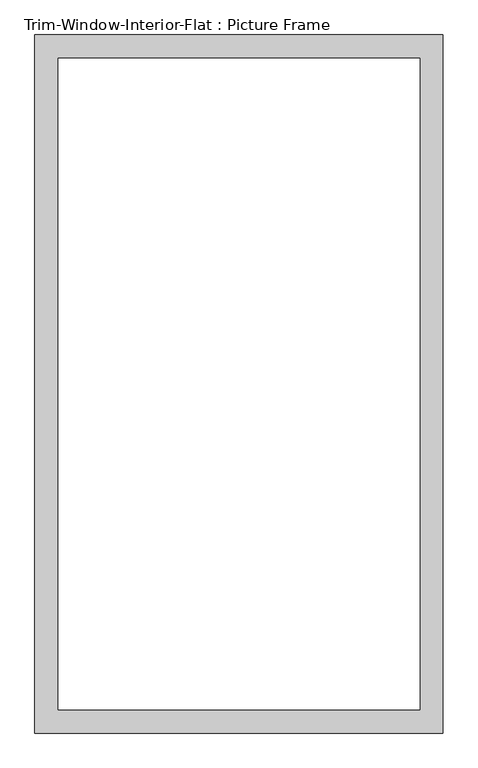
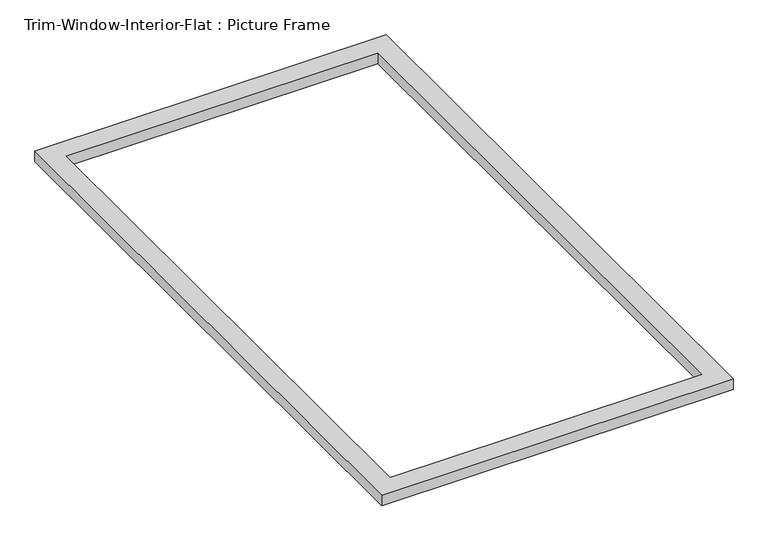
"""IFC4 building model written with IfcOpenShell, lengths in millimetres: proxy geometry, Trim-Window-Interior-Flat : Picture Frame."""

import ifcopenshell
import ifcopenshell.guid

model = None  # the IFC model being written
_history = None  # IfcOwnerHistory: only IFC2X3 demands one
_inside = {}  # id of a spatial element -> (the spatial element, [elements in it])
_under = {}  # id of a project, library or spatial element -> (it, [spatial elements below it])
_declared = {}  # id of a project -> (the project, [libraries it declares])
_typed = {}  # id of a type object -> (the type object, [elements of that type])
_made_of = {}  # id of a material, layer set ... -> (it, [elements and type objects made of it])


def new_model(schema):
    """Start an empty IFC model of exactly this schema.

    Asked for "IFC4X3", IfcOpenShell would pick the latest addendum, in which some entities
    have other attributes; the version numbers below select the first issue.
    IFC2X3 requires an IfcOwnerHistory on every rooted entity: one is made here for all.
    """
    global model, _history
    if schema == "IFC4X3":
        model = ifcopenshell.file(schema_version=(4, 3, 0, 0))
    else:
        model = ifcopenshell.file(schema=schema)
    _inside.clear()
    _under.clear()
    _declared.clear()
    _typed.clear()
    _made_of.clear()
    _history = None
    if model.schema == "IFC2X3":
        org = make("IfcOrganization", Name="unknown")
        user = make(
            "IfcPersonAndOrganization",
            ThePerson=make("IfcPerson", FamilyName="unknown"),
            TheOrganization=org,
        )
        app = make(
            "IfcApplication",
            ApplicationDeveloper=org,
            Version="unknown",
            ApplicationFullName="unknown",
            ApplicationIdentifier="unknown",
        )
        _history = make(
            "IfcOwnerHistory",
            OwningUser=user,
            OwningApplication=app,
            ChangeAction="ADDED",
            CreationDate=0,
        )
    return model


def make(cls, **values):
    """One entity of the class cls with the attributes given. An attribute that is None is left unset."""
    return model.create_entity(
        cls, **{name: value for name, value in values.items() if value is not None}
    )


def rooted(cls, **values):
    """An entity with a GlobalId (a new one), such as an element, a storey or a relation."""
    return make(cls, GlobalId=ifcopenshell.guid.new(), OwnerHistory=_history, **values)


def si_unit(unit_type, name, prefix=None):
    """IfcSIUnit, for example si_unit("LENGTHUNIT", "METRE", prefix="MILLI")."""
    return make("IfcSIUnit", UnitType=unit_type, Prefix=prefix, Name=name)


def assignment(units):
    """IfcUnitAssignment: the units of a project."""
    return None if units is None else make("IfcUnitAssignment", Units=units)


def point(xyz):
    """IfcCartesianPoint."""
    return None if xyz is None else make("IfcCartesianPoint", Coordinates=xyz)


def direction(xyz):
    """IfcDirection."""
    return None if xyz is None else make("IfcDirection", DirectionRatios=xyz)


def frame(location, z_axis=None, x_axis=None):
    """IfcAxis2Placement3D, a coordinate frame: its origin and axes. An axis left out is left unset."""
    return make(
        "IfcAxis2Placement3D",
        Location=point(location),
        Axis=direction(z_axis),
        RefDirection=direction(x_axis),
    )


def origin():
    """The frame at (0, 0, 0) with its axes left unset."""
    return frame((0.0, 0.0, 0.0))


def origin_with_axes():
    """The frame at (0, 0, 0) with the z axis (0, 0, 1) and the x axis (1, 0, 0) written out."""
    return frame((0.0, 0.0, 0.0), z_axis=(0.0, 0.0, 1.0), x_axis=(1.0, 0.0, 0.0))


def place(relative_to, where):
    """IfcLocalPlacement: puts the frame where relative to a parent placement (None: the world)."""
    return make(
        "IfcLocalPlacement", PlacementRelTo=relative_to, RelativePlacement=where
    )


def context(
    kind, dimensions, precision=None, world=None, true_north=None, identifier=None
):
    """IfcGeometricRepresentationContext, for example the 3D "Model" context."""
    return make(
        "IfcGeometricRepresentationContext",
        ContextIdentifier=identifier,
        ContextType=kind,
        CoordinateSpaceDimension=dimensions,
        Precision=precision,
        WorldCoordinateSystem=world,
        TrueNorth=true_north,
    )


def project(units=None, contexts=None):
    """IfcProject with its units and contexts."""
    return rooted(
        "IfcProject",
        Name="project",
        RepresentationContexts=contexts,
        UnitsInContext=assignment(units),
    )


def spatial(cls, under=None, at=None, **own):
    """A site, building, storey or space (cls), placed at a placement, below another one or the project."""
    s = rooted(cls, ObjectPlacement=at, **own)
    if under is not None:
        _under.setdefault(under.id(), (under, []))[1].append(s)
    return s


def polyline(points):
    """IfcPolyline through the points."""
    return make("IfcPolyline", Points=[point(p) for p in points])


def outline(outer, holes=None, kind="AREA"):
    """IfcArbitraryClosedProfileDef: a profile drawn as a closed curve; with holes, ...WithVoids."""
    if holes is None:
        return make("IfcArbitraryClosedProfileDef", ProfileType=kind, OuterCurve=outer)
    return make(
        "IfcArbitraryProfileDefWithVoids",
        ProfileType=kind,
        OuterCurve=outer,
        InnerCurves=holes,
    )


def extrude(swept, where, along, depth):
    """IfcExtrudedAreaSolid: the profile swept, set in the frame where, extruded along a direction by depth."""
    return make(
        "IfcExtrudedAreaSolid",
        SweptArea=swept,
        Position=where,
        ExtrudedDirection=direction(along),
        Depth=depth,
    )


def shape(context_of_items, identifier, shape_type, items):
    """IfcShapeRepresentation: the items that make up one representation, for example the "Body"."""
    return make(
        "IfcShapeRepresentation",
        ContextOfItems=context_of_items,
        RepresentationIdentifier=identifier,
        RepresentationType=shape_type,
        Items=items,
    )


def source(mapping_origin, context_of_items, identifier, shape_type, items):
    """IfcRepresentationMap: a shape defined once, which mapped items show again and again."""
    return make(
        "IfcRepresentationMap",
        MappingOrigin=mapping_origin,
        MappedRepresentation=shape(context_of_items, identifier, shape_type, items),
    )


def transform(
    local_origin,
    x_axis=None,
    y_axis=None,
    z_axis=None,
    scale=None,
    scale2=None,
    scale3=None,
    uniform=True,
):
    """IfcCartesianTransformationOperator3D, or its non-uniform kind. x_axis, y_axis, z_axis: its Axis1, 2, 3."""
    if uniform:
        return make(
            "IfcCartesianTransformationOperator3D",
            Axis1=direction(x_axis),
            Axis2=direction(y_axis),
            LocalOrigin=point(local_origin),
            Scale=scale,
            Axis3=direction(z_axis),
        )
    return make(
        "IfcCartesianTransformationOperator3DnonUniform",
        Axis1=direction(x_axis),
        Axis2=direction(y_axis),
        LocalOrigin=point(local_origin),
        Scale=scale,
        Axis3=direction(z_axis),
        Scale2=scale2,
        Scale3=scale3,
    )


def mapped(mapping_source, mapping_target):
    """IfcMappedItem: shows the shape of a source again, moved by a transform."""
    return make(
        "IfcMappedItem", MappingSource=mapping_source, MappingTarget=mapping_target
    )


def made_of(thing, what):
    """Note that an element or type object is made of a material, layer set ...; save() writes the relation."""
    if what is not None:
        _made_of.setdefault(what.id(), (what, []))[1].append(thing)
    return thing


def element(
    cls,
    number,
    at=None,
    inside=None,
    cuts=None,
    type_object=None,
    material=None,
    context=None,
    identifier="Body",
    shape_type=None,
    held_by="IfcProductDefinitionShape",
    body=None,
    shapes=None,
    **own,
):
    """One element of the class cls, such as IfcWall. Its Tag is "e" and its number.

    at: its placement. inside: the storey or other place that contains it. cuts: it is an
    opening in that element (IfcRelVoidsElement). A single representation is given by context,
    identifier, shape_type and body (its items); several are given by shapes. held_by: the class
    of the entity that holds the representations. save() writes the other relations.
    """
    e = rooted(cls, Tag="e%d" % number, ObjectPlacement=at, **own)
    if body is not None:
        shapes = [shape(context, identifier, shape_type, body)]
    if shapes is not None:
        e.Representation = make(held_by, Representations=shapes)
    if inside is not None:
        _inside.setdefault(inside.id(), (inside, []))[1].append(e)
    if cuts is not None:
        rooted(
            "IfcRelVoidsElement", RelatingBuildingElement=cuts, RelatedOpeningElement=e
        )
    if type_object is not None:
        _typed.setdefault(type_object.id(), (type_object, []))[1].append(e)
    return made_of(e, material)


def aggregate(whole, parts):
    """IfcRelAggregates: a whole, such as a stair, and the parts it consists of."""
    return rooted("IfcRelAggregates", RelatingObject=whole, RelatedObjects=parts)


def save(model, path):
    """Write the relations noted so far, then the file.

    IfcRelAggregates (storeys below a building ...), IfcRelContainedInSpatialStructure (elements
    in a storey), IfcRelDefinesByType, IfcRelAssociatesMaterial and IfcRelDeclares: one each for
    every whole, place, type object, material and project.
    """
    for whole, parts in _under.values():
        aggregate(whole, parts)
    for where, things in _inside.values():
        rooted(
            "IfcRelContainedInSpatialStructure",
            RelatedElements=things,
            RelatingStructure=where,
        )
    for kind, things in _typed.values():
        rooted("IfcRelDefinesByType", RelatedObjects=things, RelatingType=kind)
    for what, things in _made_of.values():
        rooted("IfcRelAssociatesMaterial", RelatedObjects=things, RelatingMaterial=what)
    for by, libraries in _declared.values():
        rooted("IfcRelDeclares", RelatingContext=by, RelatedDefinitions=libraries)
    model.write(path)


def trim_window_interior_flat_picture_frame_9b9b1be9(model_context):
    return source(origin(), model_context, "Body", "SweptSolid", [
        extrude(outline(polyline([(501.65, 44.45), (501.65, -1670.05), (-501.65, -1670.05), (-501.65, 44.45), (501.65, 44.45)]), holes=[polyline([(444.5, -12.7), (-444.5, -12.7), (-444.5, -1612.9), (444.5, -1612.9), (444.5, -12.7)])]), origin_with_axes(), (0.0, 0.0, 1.0), 31.75),
    ])


if __name__ == "__main__":
    model = new_model("IFC4")
    model_context = context("Model", 3, world=origin())
    ifc_project = project(units=[si_unit("LENGTHUNIT", "METRE", prefix="MILLI")], contexts=[model_context])
    site = spatial("IfcSite", under=ifc_project)
    building = spatial("IfcBuilding", under=site)
    placement = place(None, origin())
    trim_window_interior_flat_picture_frame_shape = trim_window_interior_flat_picture_frame_9b9b1be9(model_context)
    element("IfcBuildingElementProxy", 1, Name="Trim-Window-Interior-Flat : Picture Frame", ObjectType="Trim-Window-Interior-Flat : Picture Frame", at=placement, inside=building, context=model_context, shape_type="MappedRepresentation", body=[
        mapped(trim_window_interior_flat_picture_frame_shape, transform((0.0, 0.0, 0.0), x_axis=(1.0, 0.0, 0.0), y_axis=(0.0, 1.0, 0.0), z_axis=(0.0, 0.0, 1.0))),
    ])
    save(model, "model.ifc")

# Revit data of these elements
# Type "Trim-Window-Interior-Flat : Picture Frame"
#   Trim Thickness_Picture Frame = 0' - 1 1/4"
#   Trim Width = 0' - 2 1/4"
#   Trim Thickness_with Sill = 0' - 0 3/4"
#   Sill Thickness = 0' - 1 1/4"
#   Opening Width [instance default] = 2' - 0"
#   Opening Height [instance default] = 3' - 0"
#   Default Elevation = 4' - 0"
#   Sill = no
#   Picture Frame = yes
#   Trim Material [instance default] = none
# Element 1 (IfcBuildingElementProxy, "Trim-Window-Interior-Flat : Picture Frame")
#   Opening Width = 3' - 0"
#   Opening Height = 5' - 4"
#   Trim Material = Wood - Stained
#   Materials on its faces: "Wood - Stained"
# Materials
#   "Wood - Stained": class "Wood", colour RGB 224 178 126, transparency 0, Cost = 0
